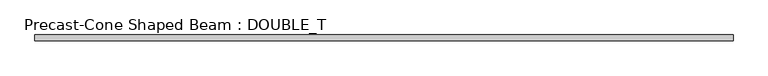
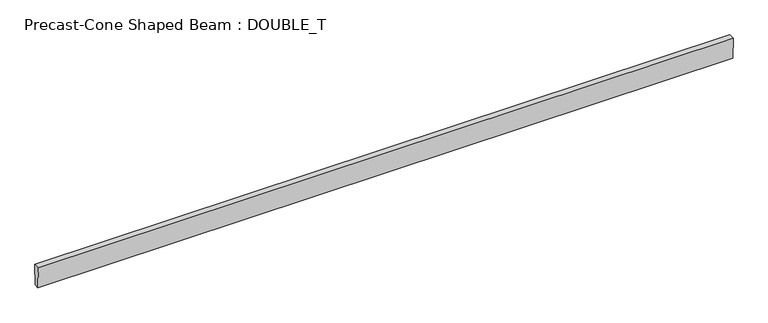
"""IFC4 building model written with IfcOpenShell, lengths in millimetres: beam geometry, Precast-Cone Shaped Beam : DOUBLE_T."""

from ifc_helpers import new_model, si_unit, frame, origin, place, context, project, spatial, polyline, outline, extrude, source, transform, mapped, element, save


def precast_cone_shaped_beam_double_t_00600c4c(model_context):
    return source(origin(), model_context, "Body", "SweptSolid", [
        extrude(outline(polyline([(50.8, -228.6), (-50.8, -228.6), (-63.5, 228.6), (63.5, 228.6), (50.8, -228.6)])), frame((-7556.5, 0.0, 0.0), z_axis=(1.0, 0.0, 0.0), x_axis=(0.0, 1.0, 0.0)), (0.0, 0.0, 1.0), 14897.1),
    ])


if __name__ == "__main__":
    model = new_model("IFC4")
    model_context = context("Model", 3, world=origin())
    ifc_project = project(units=[si_unit("LENGTHUNIT", "METRE", prefix="MILLI")], contexts=[model_context])
    site = spatial("IfcSite", under=ifc_project)
    building = spatial("IfcBuilding", under=site)
    placement = place(None, origin())
    precast_cone_shaped_beam_double_t_shape = precast_cone_shaped_beam_double_t_00600c4c(model_context)
    element("IfcBeam", 1, ObjectType="Precast-Cone Shaped Beam : DOUBLE_T", at=placement, inside=building, context=model_context, shape_type="MappedRepresentation", body=[
        mapped(precast_cone_shaped_beam_double_t_shape, transform((0.0, 0.0, 0.0), x_axis=(1.0, 0.0, 0.0), y_axis=(0.0, 1.0, 0.0), z_axis=(0.0, 0.0, 1.0))),
    ])
    save(model, "model.ifc")

# Revit data of these elements
# Type "Precast-Cone Shaped Beam : DOUBLE_T"
#   Top Width = 0' - 5"
#   Tie Rod Weight [instance default] = 30
#   Tie Rod W [instance default] = 0.0660938 kip
#   Single Rebar Weight [instance default] = 50
#   Single Rebar W [instance default] = 0.110156 kip
#   Rebar Grids Weight [instance default] = 100
#   Rebar Grids W [instance default] = 0.220313 kip
#   Depth = 1' - 6"
#   Bottom Width = 0' - 4"
#   Length [instance default] = 5' - 0"
#   Structural Material [instance default] = Concrete, Precast
#   Assembly Code = ""
# Element 1 (IfcBeam, "Precast-Cone Shaped Beam : DOUBLE_T")
#   Length = 49' - 3"
#   Structural Material = Concrete - Precast Concrete - Normal Weight Concrete - 5 ksi
#   Materials on its faces: "Concrete - Precast Concrete - Normal Weight Concrete - 5 ksi"
# Materials
#   "Concrete, Precast": class "Concrete", colour RGB 198 187 187, transparency 0, Description = "Precast concrete", Cost = 0
#   "Concrete - Precast Concrete - Normal Weight Concrete - 5 ksi": class "Concrete", colour RGB 198 187 187, transparency 0, Cost = 0
